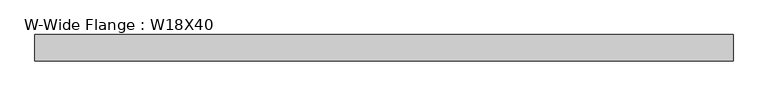
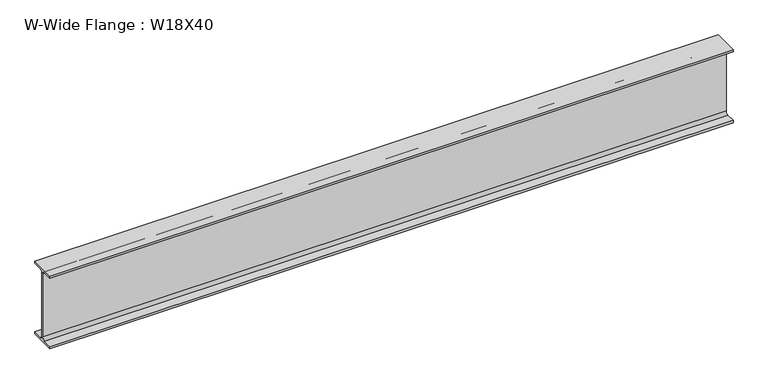
"""IFC4 building model written with IfcOpenShell, lengths in millimetres: beam geometry, W-Wide Flange : W18X40."""

from ifc_helpers import new_model, si_unit, point, frame, frame_2d, origin, place, context, project, spatial, polyline, circle_curve, trimmed, segment, composite_curve, outline, extrude, source, transform, mapped, element, save


def w_wide_flange_w18x40_6b8dc20d(model_context):
    return source(origin(), model_context, "Body", "SweptSolid", [
        extrude(outline(composite_curve([segment(polyline([(76.454, -213.995), (76.454, -227.33), (-76.454, -227.33), (-76.454, -213.995), (-20.828, -213.995)]), True, "CONTINUOUS"), segment(trimmed(circle_curve(frame_2d((-20.828, -197.1675)), 16.8275), [point((-20.828, -213.995))], [point((-4.0005, -197.1675))], True, "CARTESIAN"), True, "CONTINUOUS"), segment(polyline([(-4.0005, -197.1675), (-4.0005, 197.1675)]), True, "CONTINUOUS"), segment(trimmed(circle_curve(frame_2d((-20.828, 197.1675)), 16.8275), [point((-4.0005, 197.1675))], [point((-20.828, 213.995))], True, "CARTESIAN"), True, "CONTINUOUS"), segment(polyline([(-20.828, 213.995), (-76.454, 213.995), (-76.454, 227.33), (76.454, 227.33), (76.454, 213.995), (20.828, 213.995)]), True, "CONTINUOUS"), segment(trimmed(circle_curve(frame_2d((20.828, 197.1675)), 16.8275), [point((20.828, 213.995))], [point((4.0005, 197.1675))], True, "CARTESIAN"), True, "CONTINUOUS"), segment(polyline([(4.0005, 197.1675), (4.0005, -197.1675)]), True, "CONTINUOUS"), segment(trimmed(circle_curve(frame_2d((20.828, -197.1675)), 16.8275), [point((4.0005, -197.1675))], [point((20.828, -213.995))], True, "CARTESIAN"), True, "CONTINUOUS"), segment(polyline([(20.828, -213.995), (76.454, -213.995)]), True, "CONTINUOUS")], self_intersect=False)), frame((-2018.03, 0.0, 0.0), z_axis=(1.0, 0.0, 0.0), x_axis=(0.0, 1.0, 0.0)), (0.0, 0.0, 1.0), 4036.06),
    ])


if __name__ == "__main__":
    model = new_model("IFC4")
    model_context = context("Model", 3, world=origin())
    ifc_project = project(units=[si_unit("LENGTHUNIT", "METRE", prefix="MILLI")], contexts=[model_context])
    site = spatial("IfcSite", under=ifc_project)
    building = spatial("IfcBuilding", under=site)
    placement = place(None, origin())
    w_wide_flange_w18x40_shape = w_wide_flange_w18x40_6b8dc20d(model_context)
    element("IfcBeam", 1, ObjectType="W-Wide Flange : W18X40", at=placement, inside=building, context=model_context, shape_type="MappedRepresentation", body=[
        mapped(w_wide_flange_w18x40_shape, transform((0.0, 0.0, 0.0), x_axis=(1.0, 0.0, 0.0), y_axis=(0.0, 1.0, 0.0), z_axis=(0.0, 0.0, 1.0))),
    ])
    save(model, "model.ifc")

# Revit data of these elements
# Type "W-Wide Flange : W18X40"
#   Assembly Code = "B10"
#   W = 40
#   Length [instance default] = 5' - 0"
#   bf = 0' - 6.02"
#   d = 1' - 5.9"
#   k = 0' - 1 3/16"
#   k2 = 0' - 0.6625"
#   tf = 0' - 0.525"
#   tw = 0' - 0.315"
#   A = 0.0819444 SF
#   Structural Material [instance default] = Steel ASTM A992
# Element 1 (IfcBeam, "W-Wide Flange : W18X40")
#   Materials on its faces: "Steel ASTM A992"
# Materials
#   "Steel ASTM A992": class "Metal", colour RGB 199 199 199, transparency 0, Description = "Structural steel 50ksi", Cost = 0
